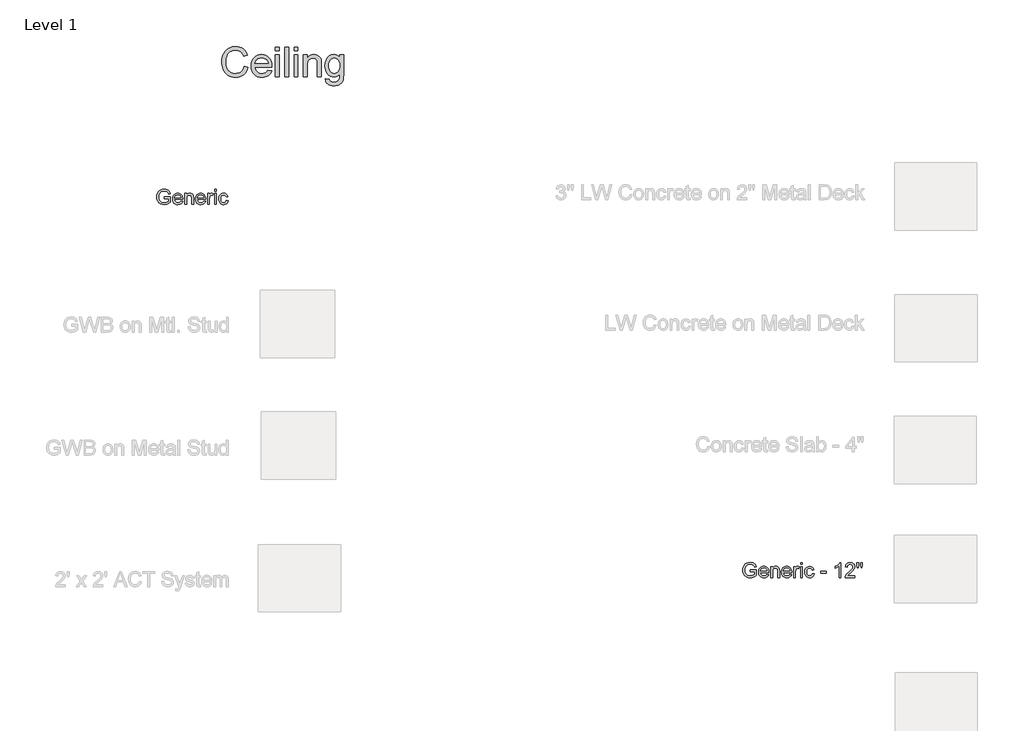
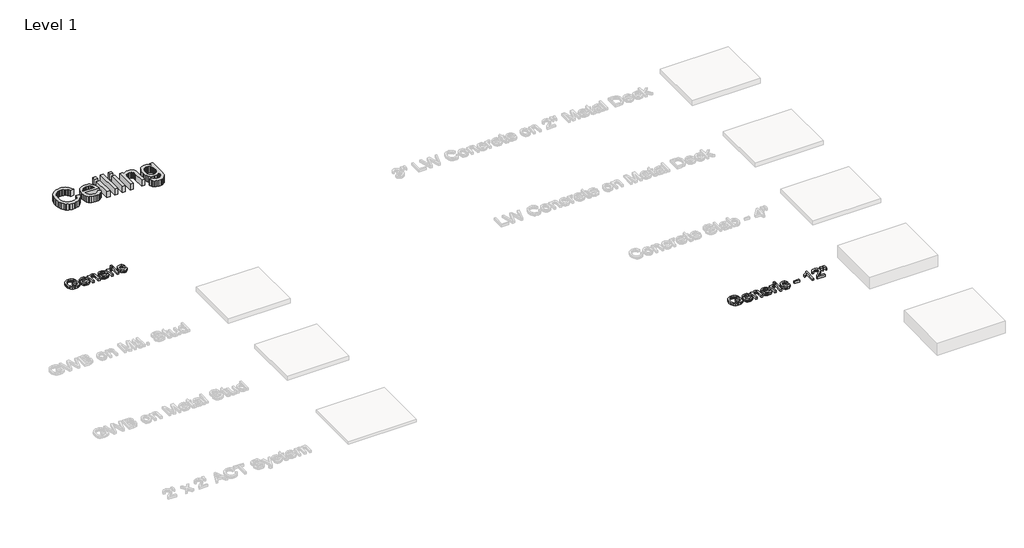
# One storey, part 12 of 42: 3 proxies.
"""IFC4 building model written with IfcOpenShell, lengths in millimetres."""

import ifcopenshell
import ifcopenshell.guid

model = None  # the IFC model being written
_history = None  # IfcOwnerHistory: only IFC2X3 demands one
_inside = {}  # id of a spatial element -> (the spatial element, [elements in it])
_under = {}  # id of a project, library or spatial element -> (it, [spatial elements below it])
_declared = {}  # id of a project -> (the project, [libraries it declares])
_typed = {}  # id of a type object -> (the type object, [elements of that type])
_made_of = {}  # id of a material, layer set ... -> (it, [elements and type objects made of it])


def new_model(schema):
    """Start an empty IFC model of exactly this schema.

    Asked for "IFC4X3", IfcOpenShell would pick the latest addendum, in which some entities
    have other attributes; the version numbers below select the first issue.
    IFC2X3 requires an IfcOwnerHistory on every rooted entity: one is made here for all.
    """
    global model, _history
    if schema == "IFC4X3":
        model = ifcopenshell.file(schema_version=(4, 3, 0, 0))
    else:
        model = ifcopenshell.file(schema=schema)
    _inside.clear()
    _under.clear()
    _declared.clear()
    _typed.clear()
    _made_of.clear()
    _history = None
    if model.schema == "IFC2X3":
        org = make("IfcOrganization", Name="unknown")
        user = make(
            "IfcPersonAndOrganization",
            ThePerson=make("IfcPerson", FamilyName="unknown"),
            TheOrganization=org,
        )
        app = make(
            "IfcApplication",
            ApplicationDeveloper=org,
            Version="unknown",
            ApplicationFullName="unknown",
            ApplicationIdentifier="unknown",
        )
        _history = make(
            "IfcOwnerHistory",
            OwningUser=user,
            OwningApplication=app,
            ChangeAction="ADDED",
            CreationDate=0,
        )
    return model


def make(cls, **values):
    """One entity of the class cls with the attributes given. An attribute that is None is left unset."""
    return model.create_entity(
        cls, **{name: value for name, value in values.items() if value is not None}
    )


def rooted(cls, **values):
    """An entity with a GlobalId (a new one), such as an element, a storey or a relation."""
    return make(cls, GlobalId=ifcopenshell.guid.new(), OwnerHistory=_history, **values)


def si_unit(unit_type, name, prefix=None):
    """IfcSIUnit, for example si_unit("LENGTHUNIT", "METRE", prefix="MILLI")."""
    return make("IfcSIUnit", UnitType=unit_type, Prefix=prefix, Name=name)


def assignment(units):
    """IfcUnitAssignment: the units of a project."""
    return None if units is None else make("IfcUnitAssignment", Units=units)


def point(xyz):
    """IfcCartesianPoint."""
    return None if xyz is None else make("IfcCartesianPoint", Coordinates=xyz)


def direction(xyz):
    """IfcDirection."""
    return None if xyz is None else make("IfcDirection", DirectionRatios=xyz)


def frame(location, z_axis=None, x_axis=None):
    """IfcAxis2Placement3D, a coordinate frame: its origin and axes. An axis left out is left unset."""
    return make(
        "IfcAxis2Placement3D",
        Location=point(location),
        Axis=direction(z_axis),
        RefDirection=direction(x_axis),
    )


def origin():
    """The frame at (0, 0, 0) with its axes left unset."""
    return frame((0.0, 0.0, 0.0))


def origin_with_axes():
    """The frame at (0, 0, 0) with the z axis (0, 0, 1) and the x axis (1, 0, 0) written out."""
    return frame((0.0, 0.0, 0.0), z_axis=(0.0, 0.0, 1.0), x_axis=(1.0, 0.0, 0.0))


def place(relative_to, where):
    """IfcLocalPlacement: puts the frame where relative to a parent placement (None: the world)."""
    return make(
        "IfcLocalPlacement", PlacementRelTo=relative_to, RelativePlacement=where
    )


def context(
    kind, dimensions, precision=None, world=None, true_north=None, identifier=None
):
    """IfcGeometricRepresentationContext, for example the 3D "Model" context."""
    return make(
        "IfcGeometricRepresentationContext",
        ContextIdentifier=identifier,
        ContextType=kind,
        CoordinateSpaceDimension=dimensions,
        Precision=precision,
        WorldCoordinateSystem=world,
        TrueNorth=true_north,
    )


def project(units=None, contexts=None):
    """IfcProject with its units and contexts."""
    return rooted(
        "IfcProject",
        Name="project",
        RepresentationContexts=contexts,
        UnitsInContext=assignment(units),
    )


def spatial(cls, under=None, at=None, **own):
    """A site, building, storey or space (cls), placed at a placement, below another one or the project."""
    s = rooted(cls, ObjectPlacement=at, **own)
    if under is not None:
        _under.setdefault(under.id(), (under, []))[1].append(s)
    return s


def polyline(points):
    """IfcPolyline through the points."""
    return make("IfcPolyline", Points=[point(p) for p in points])


def outline(outer, holes=None, kind="AREA"):
    """IfcArbitraryClosedProfileDef: a profile drawn as a closed curve; with holes, ...WithVoids."""
    if holes is None:
        return make("IfcArbitraryClosedProfileDef", ProfileType=kind, OuterCurve=outer)
    return make(
        "IfcArbitraryProfileDefWithVoids",
        ProfileType=kind,
        OuterCurve=outer,
        InnerCurves=holes,
    )


def extrude(swept, where, along, depth):
    """IfcExtrudedAreaSolid: the profile swept, set in the frame where, extruded along a direction by depth."""
    return make(
        "IfcExtrudedAreaSolid",
        SweptArea=swept,
        Position=where,
        ExtrudedDirection=direction(along),
        Depth=depth,
    )


def shape(context_of_items, identifier, shape_type, items):
    """IfcShapeRepresentation: the items that make up one representation, for example the "Body"."""
    return make(
        "IfcShapeRepresentation",
        ContextOfItems=context_of_items,
        RepresentationIdentifier=identifier,
        RepresentationType=shape_type,
        Items=items,
    )


def made_of(thing, what):
    """Note that an element or type object is made of a material, layer set ...; save() writes the relation."""
    if what is not None:
        _made_of.setdefault(what.id(), (what, []))[1].append(thing)
    return thing


def element(
    cls,
    number,
    at=None,
    inside=None,
    cuts=None,
    type_object=None,
    material=None,
    context=None,
    identifier="Body",
    shape_type=None,
    held_by="IfcProductDefinitionShape",
    body=None,
    shapes=None,
    **own,
):
    """One element of the class cls, such as IfcWall. Its Tag is "e" and its number.

    at: its placement. inside: the storey or other place that contains it. cuts: it is an
    opening in that element (IfcRelVoidsElement). A single representation is given by context,
    identifier, shape_type and body (its items); several are given by shapes. held_by: the class
    of the entity that holds the representations. save() writes the other relations.
    """
    e = rooted(cls, Tag="e%d" % number, ObjectPlacement=at, **own)
    if body is not None:
        shapes = [shape(context, identifier, shape_type, body)]
    if shapes is not None:
        e.Representation = make(held_by, Representations=shapes)
    if inside is not None:
        _inside.setdefault(inside.id(), (inside, []))[1].append(e)
    if cuts is not None:
        rooted(
            "IfcRelVoidsElement", RelatingBuildingElement=cuts, RelatedOpeningElement=e
        )
    if type_object is not None:
        _typed.setdefault(type_object.id(), (type_object, []))[1].append(e)
    return made_of(e, material)


def aggregate(whole, parts):
    """IfcRelAggregates: a whole, such as a stair, and the parts it consists of."""
    return rooted("IfcRelAggregates", RelatingObject=whole, RelatedObjects=parts)


def save(model, path):
    """Write the relations noted so far, then the file.

    IfcRelAggregates (storeys below a building ...), IfcRelContainedInSpatialStructure (elements
    in a storey), IfcRelDefinesByType, IfcRelAssociatesMaterial and IfcRelDeclares: one each for
    every whole, place, type object, material and project.
    """
    for whole, parts in _under.values():
        aggregate(whole, parts)
    for where, things in _inside.values():
        rooted(
            "IfcRelContainedInSpatialStructure",
            RelatedElements=things,
            RelatingStructure=where,
        )
    for kind, things in _typed.values():
        rooted("IfcRelDefinesByType", RelatedObjects=things, RelatingType=kind)
    for what, things in _made_of.values():
        rooted("IfcRelAssociatesMaterial", RelatedObjects=things, RelatingMaterial=what)
    for by, libraries in _declared.values():
        rooted("IfcRelDeclares", RelatingContext=by, RelatedDefinitions=libraries)
    model.write(path)


model = new_model("IFC4")

# Units and contexts
model_context = context("Model", 3, world=origin())
ifc_project = project(units=[si_unit("LENGTHUNIT", "METRE", prefix="MILLI")], contexts=[model_context])

# Site, building, storey
site = spatial("IfcSite", under=ifc_project)
building = spatial("IfcBuilding", under=site)
storey = spatial("IfcBuildingStorey", under=building, Name="Level 1", Elevation=0.0)

# Proxies
placement = place(None, origin())
element("IfcBuildingElementProxy", 1, Name="24\" Arial", ObjectType="24\" Arial", at=placement, inside=storey, context=model_context, shape_type="SweptSolid", body=[
    extrude(outline(polyline([(10519.6706073, -3278.5487239), (10595.8123808, -3298.1790249), (10580.745753, -3345.5306198), (10560.6786034, -3386.9057546), (10535.6109322, -3422.3044295), (10505.5427391, -3451.7266444), (10471.1525338, -3474.8563811), (10433.1188256, -3491.3776216), (10391.4416147, -3501.2903659), (10346.1209008, -3504.5946141), (10299.6894763, -3502.0943532), (10257.8031357, -3494.5935706), (10220.461879, -3482.0922662), (10187.6657061, -3464.5904401), (10158.9638267, -3442.3483424), (10133.90545, -3415.6262234), (10112.4905762, -3384.4240831), (10094.7192053, -3348.7419214), (10080.7632882, -3310.1226503), (10070.7947759, -3270.1091816), (10064.8136686, -3228.7015155), (10062.8199662, -3185.8996518), (10065.0739188, -3139.9747858), (10071.8357767, -3097.0799756), (10083.10554, -3057.2152214), (10098.8832085, -3020.3805231), (10118.8155856, -2987.1846803), (10142.5494746, -2958.2364926), (10170.0848755, -2933.53596), (10201.4217883, -2913.0830825), (10235.4959755, -2897.0451638), (10271.2431997, -2885.5895075), (10308.663461, -2878.7161138), (10347.7567592, -2876.4249825), (10391.3068422, -2879.3899759), (10431.2413063, -2888.284956), (10467.5601515, -2903.1099229), (10500.2633779, -2923.8648766), (10528.8118956, -2950.0014326), (10552.6666151, -2980.9712067), (10571.8275362, -3016.7741989), (10586.2946591, -3057.410409), (10510.1528856, -3075.553566), (10498.162787, -3045.6108508), (10483.7560793, -3020.0273264), (10466.9327627, -2998.8029929), (10447.692837, -2981.9378503), (10425.9247665, -2969.0879966), (10401.5170153, -2959.9095296), (10374.4695836, -2954.4024494), (10344.7824712, -2952.5667561), (10310.6246321, -2954.6022844), (10279.3853132, -2960.7088695), (10251.0645144, -2970.8865114), (10225.6622357, -2985.13521), (10203.4991426, -3002.8136344), (10184.8959004, -3023.2804539), (10169.8525092, -3046.5356684), (10158.3689691, -3072.579278), (10143.813547, -3128.3099999), (10138.9617397, -3185.7509374), (10144.7058334, -3256.0928493), (10151.8859506, -3287.6946596), (10161.9381147, -3316.9170395), (10175.024982, -3343.1790733), (10191.309209, -3365.8998454), (10210.7907956, -3385.0793559), (10233.4697418, -3400.7176047), (10258.2446316, -3412.8517704), (10284.0140489, -3421.5190316), (10310.7779939, -3426.7193883), (10338.5364664, -3428.4528405), (10371.6393626, -3426.0919994), (10402.0932837, -3419.009476), (10429.8982294, -3407.2052704), (10455.0541999, -3390.6793826), (10476.9663374, -3369.5061697), (10495.0397845, -3343.7599889), (10509.2745411, -3313.4408404), (10519.6706073, -3278.5487239)])), origin_with_axes(), (0.0, 0.0, 1.0), 152.4),
    extrude(outline(polyline([(11004.182127, -3361.8287887), (11078.8367565, -3371.3465104), (11067.3903949, -3401.2473997), (11051.9380392, -3427.5977327), (11032.4796892, -3450.3975094), (11009.0153451, -3469.6467297), (10981.7866676, -3484.9364291), (10951.0353178, -3495.857643), (10916.7612956, -3502.4103713), (10878.964601, -3504.5946141), (10831.7198946, -3500.8256334), (10789.6244244, -3489.5186916), (10752.6781903, -3470.6737886), (10720.8811924, -3444.2909243), (10695.31161, -3411.1043761), (10677.0476225, -3371.8484215), (10666.0892301, -3326.5230603), (10662.4364326, -3275.1282927), (10666.1264087, -3221.9907781), (10677.1963369, -3175.1550363), (10695.6462174, -3134.6210673), (10721.47605, -3100.388871), (10753.1893961, -3073.1927249), (10789.289817, -3053.7669062), (10829.7773128, -3042.111415), (10874.6518834, -3038.2262513), (10918.0811359, -3042.1021203), (10957.3556799, -3053.7297276), (10992.4755152, -3073.109073), (11023.440642, -3100.2401566), (11048.7174429, -3134.3979957), (11066.7723007, -3174.8576075), (11077.6052154, -3221.6189921), (11081.2161869, -3274.6821495), (11080.7700437, -3295.2047369), (10738.5782061, -3295.2047369), (10742.9885176, -3325.588948), (10751.7580199, -3352.1995312), (10764.8867132, -3375.0364865), (10782.3745973, -3394.0998138), (10803.2550288, -3409.129263), (10826.5613639, -3419.8645839), (10852.2936026, -3426.3057764), (10880.4517451, -3428.4528405), (10920.9764194, -3424.4747303), (10955.1063746, -3412.5403996), (10982.8416104, -3391.9062764), (11004.182127, -3361.8287887)]), holes=[polyline([(10738.5782061, -3219.0629634), (11005.0744134, -3219.0629634), (10994.7759411, -3178.8357178), (10985.9181396, -3163.0162233), (10974.5879611, -3150.0594811), (10953.8237128, -3134.444469), (10930.1967123, -3123.2908889), (10903.7069596, -3116.5987408), (10874.3544546, -3114.3680248), (10847.581215, -3116.1479503), (10823.0293968, -3121.4877267), (10800.699, -3130.3873542), (10780.5900245, -3142.8468326), (10763.7155873, -3158.2898938), (10751.0888051, -3176.1402693), (10742.7096781, -3196.3979591), (10738.5782061, -3219.0629634)])]), origin_with_axes(), (0.0, 0.0, 1.0), 152.4),
    extrude(outline(polyline([(11157.3579605, -2962.0844777), (11157.3579605, -2885.9427042), (11233.499734, -2885.9427042), (11233.499734, -2962.0844777), (11157.3579605, -2962.0844777)])), origin_with_axes(), (0.0, 0.0, 1.0), 152.4),
    extrude(outline(polyline([(11157.3579605, -3495.0768924), (11157.3579605, -3047.7439729), (11233.499734, -3047.7439729), (11233.499734, -3495.0768924), (11157.3579605, -3495.0768924)])), origin_with_axes(), (0.0, 0.0, 1.0), 152.4),
    extrude(outline(polyline([(11347.7123943, -3495.0768924), (11347.7123943, -2885.9427042), (11423.8541678, -2885.9427042), (11423.8541678, -3495.0768924), (11347.7123943, -3495.0768924)])), origin_with_axes(), (0.0, 0.0, 1.0), 152.4),
    extrude(outline(polyline([(11538.0668281, -2962.0844777), (11538.0668281, -2885.9427042), (11614.2086016, -2885.9427042), (11614.2086016, -2962.0844777), (11538.0668281, -2962.0844777)])), origin_with_axes(), (0.0, 0.0, 1.0), 152.4),
    extrude(outline(polyline([(11538.0668281, -3495.0768924), (11538.0668281, -3047.7439729), (11614.2086016, -3047.7439729), (11614.2086016, -3495.0768924), (11538.0668281, -3495.0768924)])), origin_with_axes(), (0.0, 0.0, 1.0), 152.4),
    extrude(outline(polyline([(11728.4212618, -3495.0768924), (11728.4212618, -3047.7439729), (11804.5630354, -3047.7439729), (11804.5630354, -3110.2040215), (11831.0156095, -3078.713747), (11862.7847235, -3056.2206938), (11899.8703774, -3042.7248619), (11942.2725711, -3038.2262513), (11979.8043681, -3041.8511648), (12014.1759841, -3052.7259054), (12042.840685, -3069.4934542), (12063.2517366, -3090.7967922), (12077.1007652, -3116.5801515), (12086.0793972, -3146.7877643), (12090.0946861, -3220.401393), (12090.0946861, -3495.0768924), (12013.9529125, -3495.0768924), (12013.9529125, -3230.6626867), (12011.7593751, -3191.2905489), (12005.1787629, -3163.2950628), (11993.0399498, -3143.2372079), (11974.1718102, -3127.6779637), (11949.9871306, -3117.6955095), (11921.8986981, -3114.3680248), (11898.778256, -3116.2362494), (11877.3029669, -3121.8409234), (11857.472831, -3131.1820468), (11839.2878481, -3144.2596195), (11824.0957425, -3162.5607855), (11813.2442385, -3187.5726889), (11806.7333362, -3219.2953296), (11804.5630354, -3257.7287077), (11804.5630354, -3495.0768924), (11728.4212618, -3495.0768924)])), origin_with_axes(), (0.0, 0.0, 1.0), 152.4),
    extrude(outline(polyline([(12175.7541813, -3533.1477791), (12251.8959548, -3542.6655008), (12260.2983185, -3566.459805), (12276.5825454, -3582.8183892), (12308.5933203, -3595.5334705), (12350.4936029, -3599.7718309), (12395.1822805, -3594.9757915), (12413.232491, -3588.9807422), (12428.4199492, -3580.5876732), (12451.4706815, -3557.5369409), (12465.5985496, -3526.7530599), (12469.7253742, -3493.998713), (12470.8035536, -3437.9705622), (12445.4663375, -3462.9545817), (12417.1920119, -3480.8003098), (12385.9805769, -3491.5077467), (12351.8320325, -3495.0768924), (12310.0851116, -3490.9221838), (12273.3294179, -3478.458058), (12241.5649512, -3457.6845151), (12214.7917116, -3428.6015549), (12193.5487888, -3393.7094385), (12178.3752726, -3355.5084266), (12169.2711628, -3313.9985194), (12166.2364596, -3269.1797166), (12171.6831245, -3207.704901), (12188.0231194, -3151.1748391), (12200.1340484, -3125.6842613), (12214.6801758, -3103.2702126), (12231.6615015, -3083.9326931), (12251.0780256, -3067.6717027), (12272.6183771, -3054.7893177), (12295.9711855, -3045.5876141), (12321.1364506, -3040.066592), (12348.1141725, -3038.2262513), (12383.721977, -3042.3902545), (12416.0394753, -3054.8822642), (12445.0666675, -3075.7022804), (12470.8035536, -3104.8503031), (12470.8035536, -3047.7439729), (12546.9453272, -3047.7439729), (12546.9453272, -3433.9552734), (12541.7403231, -3523.1281463), (12535.234068, -3556.2961052), (12526.125311, -3581.8517456), (12514.1956276, -3602.4626321), (12499.2265936, -3620.7963294), (12481.2182091, -3636.8528375), (12460.1704739, -3650.6321562), (12436.2971652, -3661.6927898), (12409.8120598, -3669.5932424), (12380.7151577, -3674.3335139), (12349.0064589, -3675.9136045), (12311.7023808, -3673.6875358), (12278.1626359, -3667.0093297), (12248.3872244, -3655.8789862), (12222.3761461, -3640.2965053), (12201.3655896, -3620.2432978), (12186.5917433, -3595.7007742), (12178.0546072, -3566.6689347), (12175.7541813, -3533.1477791)]), holes=[polyline([(12242.3782331, -3263.9747126), (12244.4091141, -3301.6226928), (12250.5017573, -3333.8147133), (12260.6561625, -3360.5507743), (12274.8723298, -3381.8308757), (12292.1557316, -3398.0639821), (12311.5118404, -3409.6590581), (12332.9406562, -3416.6161036), (12356.442179, -3418.9351188), (12379.7113355, -3416.6300456), (12401.0379101, -3409.714826), (12420.4219028, -3398.1894598), (12437.8633137, -3382.0539473), (12452.2746687, -3360.9829755), (12462.5684937, -3334.6512319), (12468.7447886, -3303.0587162), (12470.8035536, -3266.2054286), (12468.6843734, -3230.8904056), (12462.3268328, -3200.1948237), (12451.7309317, -3174.1186829), (12436.8966701, -3152.6619831), (12419.0788259, -3135.9083764), (12399.5321768, -3123.9415144), (12378.2567227, -3116.7613972), (12355.2524637, -3114.3680248), (12332.6339328, -3116.7242186), (12311.7720906, -3123.7928), (12292.6669374, -3135.573769), (12275.318473, -3152.0671255), (12260.907118, -3173.1985125), (12250.6132931, -3198.8935727), (12244.4369981, -3229.152306), (12242.3782331, -3263.9747126)])]), origin_with_axes(), (0.0, 0.0, 1.0), 152.4),
])
element("IfcBuildingElementProxy", 2, Name="8\" Arial", ObjectType="8\" Arial", at=placement, inside=storey, context=model_context, shape_type="SweptSolid", body=[
    extrude(outline(polyline([(8891.7639138, -5976.3008915), (8891.7639138, -5938.2300048), (9015.4942958, -5938.2300048), (9015.4942958, -6052.070879), (8985.4261028, -6072.9838417), (8954.4098554, -6087.985407), (8922.519911, -6097.0198069), (8889.8306266, -6100.0312735), (8847.1217095, -6095.2445287), (8808.5210276, -6080.8842943), (8776.4544848, -6057.4524814), (8753.3479847, -6025.4510012), (8739.3781256, -5987.0640963), (8734.721506, -5944.4760096), (8739.3595363, -5901.5811995), (8753.2736275, -5861.6792666), (8775.8875112, -5828.2092317), (8790.2407746, -5815.1758086), (8806.624919, -5804.6101151), (8844.0637696, -5790.6123721), (8886.7819814, -5785.9464577), (8918.1421308, -5788.6512009), (8946.3420991, -5796.7654304), (8970.0899301, -5809.7035834), (8988.0936673, -5826.8800967), (9001.4129009, -5849.1221944), (9011.107221, -5877.2571002), (8976.0106222, -5887.1466079), (8968.1752322, -5867.0794584), (8958.6482159, -5851.9384734), (8946.0446703, -5840.5246431), (8928.9796928, -5831.6389576), (8908.6337037, -5825.9227478), (8886.1871238, -5824.0173445), (8859.911148, -5826.0714622), (8837.4459787, -5832.2338152), (8818.8752678, -5841.7329476), (8804.2826672, -5853.7974034), (8784.6895448, -5883.1313191), (8775.7666807, -5911.8703771), (8772.7923927, -5942.9145084), (8776.370833, -5979.3216528), (8787.1061538, -6009.27831), (8804.6730425, -6032.5707032), (8828.7461862, -6048.9850552), (8856.9182707, -6058.7165539), (8886.7819814, -6061.9603867), (8913.1509037, -6059.5158938), (8938.8692005, -6052.1824148), (8961.2042446, -6042.0791302), (8977.423409, -6031.32522), (8977.423409, -5976.3008915), (8891.7639138, -5976.3008915)])), origin_with_axes(), (0.0, 0.0, 1.0), 50.8),
    extrude(outline(polyline([(9229.1968906, -6028.6483608), (9266.5242054, -6033.4072217), (9253.0748467, -6061.5328328), (9231.6134996, -6082.5573313), (9202.623486, -6095.662788), (9166.5881276, -6100.0312735), (9142.9657744, -6098.1467832), (9121.9180393, -6092.4933123), (9103.4449223, -6083.0708607), (9087.5464233, -6069.8794286), (9074.7616321, -6053.2861545), (9065.6296384, -6033.6581772), (9060.1504421, -6010.9954966), (9058.3240434, -5985.2981128), (9060.1690314, -5958.7293555), (9065.7039956, -5935.3114846), (9074.9289358, -5915.0445001), (9087.8438521, -5897.928402), (9103.7005251, -5884.3303289), (9121.7507356, -5874.6174196), (9141.9944835, -5868.789674), (9164.4317688, -5866.8470921), (9186.1463951, -5868.7850266), (9205.783667, -5874.5988303), (9223.3435847, -5884.288503), (9238.8261481, -5897.8540448), (9251.4645486, -5914.9329643), (9260.4919775, -5935.1627702), (9265.9084348, -5958.5434625), (9267.7139206, -5985.0750412), (9267.490849, -5995.3363349), (9096.3949302, -5995.3363349), (9102.9848371, -6023.8337321), (9118.2931258, -6044.7838734), (9140.386509, -6057.6662584), (9167.3316996, -6061.9603867), (9187.5940368, -6059.9713316), (9204.6590144, -6054.0041663), (9218.5266323, -6043.6871047), (9229.1968906, -6028.6483608)]), holes=[polyline([(9096.3949302, -5957.2654481), (9229.6430338, -5957.2654481), (9224.4937977, -5937.1518254), (9214.3998077, -5922.763707), (9192.2041833, -5909.3794109), (9164.2830544, -5904.9179789), (9138.6205255, -5908.4778298), (9117.4008394, -5919.1573828), (9102.6502297, -5935.8041011), (9096.3949302, -5957.2654481)])]), origin_with_axes(), (0.0, 0.0, 1.0), 50.8),
    extrude(outline(polyline([(9305.7848073, -6095.2724126), (9305.7848073, -5871.6059529), (9343.8556941, -5871.6059529), (9343.8556941, -5902.8359772), (9357.0819812, -5887.09084), (9372.9665382, -5875.8443134), (9391.5093651, -5869.0963974), (9412.7104619, -5866.8470921), (9431.4763605, -5868.6595489), (9448.6621685, -5874.0969192), (9462.9945189, -5882.4806935), (9473.2000447, -5893.1323625), (9484.613875, -5921.1278486), (9486.6215194, -5957.934663), (9486.6215194, -6095.2724126), (9448.5506327, -6095.2724126), (9448.5506327, -5963.0653098), (9444.1635578, -5929.3814979), (9438.0941513, -5919.3525704), (9428.6600815, -5911.5729483), (9416.5677417, -5906.5817212), (9402.5235254, -5904.9179789), (9380.2256599, -5908.6544282), (9361.2181005, -5919.8637762), (9353.6220477, -5929.0143592), (9348.1962957, -5941.5203109), (9343.8556941, -5976.5983203), (9343.8556941, -6095.2724126), (9305.7848073, -6095.2724126)])), origin_with_axes(), (0.0, 0.0, 1.0), 50.8),
    extrude(outline(polyline([(9695.5652534, -6028.6483608), (9732.8925682, -6033.4072217), (9719.4432095, -6061.5328328), (9697.9818624, -6082.5573313), (9668.9918488, -6095.662788), (9632.9564904, -6100.0312735), (9609.3341372, -6098.1467832), (9588.2864021, -6092.4933123), (9569.813285, -6083.0708607), (9553.9147861, -6069.8794286), (9541.1299949, -6053.2861545), (9531.9980012, -6033.6581772), (9526.5188049, -6010.9954966), (9524.6924062, -5985.2981128), (9526.5373942, -5958.7293555), (9532.0723584, -5935.3114846), (9541.2972986, -5915.0445001), (9554.2122149, -5897.928402), (9570.0688879, -5884.3303289), (9588.1190984, -5874.6174196), (9608.3628463, -5868.789674), (9630.8001316, -5866.8470921), (9652.5147579, -5868.7850266), (9672.1520298, -5874.5988303), (9689.7119475, -5884.288503), (9705.1945109, -5897.8540448), (9717.8329113, -5914.9329643), (9726.8603402, -5935.1627702), (9732.2767976, -5958.5434625), (9734.0822834, -5985.0750412), (9733.8592118, -5995.3363349), (9562.763293, -5995.3363349), (9569.3531999, -6023.8337321), (9584.6614886, -6044.7838734), (9606.7548718, -6057.6662584), (9633.7000624, -6061.9603867), (9653.9623996, -6059.9713316), (9671.0273772, -6054.0041663), (9684.8949951, -6043.6871047), (9695.5652534, -6028.6483608)]), holes=[polyline([(9562.763293, -5957.2654481), (9696.0113966, -5957.2654481), (9690.8621605, -5937.1518254), (9680.7681705, -5922.763707), (9658.5725461, -5909.3794109), (9630.6514172, -5904.9179789), (9604.9888883, -5908.4778298), (9583.7692021, -5919.1573828), (9569.0185925, -5935.8041011), (9562.763293, -5957.2654481)])]), origin_with_axes(), (0.0, 0.0, 1.0), 50.8),
    extrude(outline(polyline([(9772.1531701, -6095.2724126), (9772.1531701, -5871.6059529), (9805.465196, -5871.6059529), (9805.465196, -5904.6949073), (9817.7713128, -5885.5107495), (9829.1107859, -5874.208455), (9840.4874376, -5868.6874328), (9852.9050901, -5866.8470921), (9871.8661763, -5869.7842015), (9891.1246912, -5878.5955298), (9878.4096099, -5912.7254849), (9865.0253138, -5906.8698554), (9851.6410177, -5904.9179789), (9840.2736606, -5906.7954982), (9830.1146081, -5912.4280561), (9821.907432, -5921.3880988), (9816.3957045, -5933.2480723), (9811.7669688, -5954.5142317), (9810.2240569, -5977.7136783), (9810.2240569, -6095.2724126), (9772.1531701, -6095.2724126)])), origin_with_axes(), (0.0, 0.0, 1.0), 50.8),
    extrude(outline(polyline([(9914.9189955, -6095.2724126), (9914.9189955, -5871.6059529), (9952.9898822, -5871.6059529), (9952.9898822, -6095.2724126), (9914.9189955, -6095.2724126)])), origin_with_axes(), (0.0, 0.0, 1.0), 50.8),
    extrude(outline(polyline([(9914.9189955, -5828.7762053), (9914.9189955, -5790.7053186), (9952.9898822, -5790.7053186), (9952.9898822, -5828.7762053), (9914.9189955, -5828.7762053)])), origin_with_axes(), (0.0, 0.0, 1.0), 50.8),
    extrude(outline(polyline([(10152.8620377, -6014.3717783), (10190.9329245, -6019.1306391), (10180.3184341, -6052.9910494), (10160.372115, -6078.5792211), (10132.9714865, -6094.6682604), (10099.994068, -6100.0312735), (10078.6419331, -6098.1607252), (10059.4972776, -6092.5490802), (10042.5601015, -6083.1963385), (10027.8304047, -6070.1025002), (10015.9076923, -6053.5138735), (10007.3914692, -6033.6767665), (10002.2817353, -6010.5911794), (10000.5784907, -5984.257112), (10003.4877162, -5950.3781124), (10012.2153926, -5921.0163128), (10026.9009397, -5897.3056604), (10047.6837773, -5880.3801026), (10072.5469663, -5870.2303447), (10099.4735676, -5866.8470921), (10131.6423516, -5871.4944171), (10157.3606484, -5885.4363923), (10175.8105288, -5907.9294455), (10186.1740636, -5938.2300048), (10148.1031769, -5942.9888656), (10141.1972518, -5926.3793259), (10130.4433417, -5914.4728791), (10116.436304, -5907.3067039), (10099.7709964, -5904.9179789), (10075.1680576, -5909.6210718), (10055.6399978, -5923.7303506), (10042.8970325, -5948.0079767), (10038.6493774, -5983.2161112), (10042.804086, -6018.8982729), (10055.2682118, -6043.2595508), (10074.4430749, -6057.2851777), (10098.7299956, -6061.9603867), (10118.4439484, -6059.0418666), (10134.6073449, -6050.2863062), (10146.3650773, -6035.470634), (10152.8620377, -6014.3717783)])), origin_with_axes(), (0.0, 0.0, 1.0), 50.8),
])
element("IfcBuildingElementProxy", 3, Name="8\" Arial", ObjectType="8\" Arial", at=placement, inside=storey, context=model_context, shape_type="SweptSolid", body=[
    extrude(outline(polyline([(20843.5857887, -13586.9353263), (20843.5857887, -13548.8644395), (20967.3161707, -13548.8644395), (20967.3161707, -13662.7053138), (20937.2479777, -13683.6182765), (20906.2317303, -13698.6198417), (20874.3417859, -13707.6542416), (20841.6525015, -13710.6657082), (20798.9435844, -13705.8789634), (20760.3429025, -13691.518729), (20728.2763597, -13668.0869162), (20705.1698596, -13636.0854359), (20691.2000005, -13597.6985311), (20686.5433808, -13555.1104444), (20691.1814112, -13512.2156342), (20705.0955024, -13472.3137014), (20727.7093861, -13438.8436664), (20742.0626495, -13425.8102433), (20758.4467939, -13415.2445498), (20795.8856445, -13401.2468068), (20838.6038563, -13396.5808925), (20869.9640057, -13399.2856356), (20898.163974, -13407.3998652), (20921.911805, -13420.3380181), (20939.9155422, -13437.5145315), (20953.2347758, -13459.7566291), (20962.9290958, -13487.8915349), (20927.8324971, -13497.7810426), (20919.9971071, -13477.7138931), (20910.4700908, -13462.5729081), (20897.8665452, -13451.1590778), (20880.8015677, -13442.2733923), (20860.4555786, -13436.5571825), (20838.0089987, -13434.6517792), (20811.7330229, -13436.7058969), (20789.2678536, -13442.8682499), (20770.6971427, -13452.3673823), (20756.1045421, -13464.4318381), (20736.5114197, -13493.7657538), (20727.5885556, -13522.5048119), (20724.6142676, -13553.5489431), (20728.1927079, -13589.9560875), (20738.9280287, -13619.9127448), (20756.4949174, -13643.2051379), (20780.5680611, -13659.6194899), (20808.7401455, -13669.3509886), (20838.6038563, -13672.5948215), (20864.9727786, -13670.1503285), (20890.6910754, -13662.8168496), (20913.0261195, -13652.7135649), (20929.2452839, -13641.9596548), (20929.2452839, -13586.9353263), (20843.5857887, -13586.9353263)])), origin_with_axes(), (0.0, 0.0, 1.0), 50.8),
    extrude(outline(polyline([(21181.0187655, -13639.2827956), (21218.3460803, -13644.0416564), (21204.8967216, -13672.1672676), (21183.4353745, -13693.1917661), (21154.4453609, -13706.2972227), (21118.4100025, -13710.6657082), (21094.7876493, -13708.7812179), (21073.7399142, -13703.127747), (21055.2667971, -13693.7052955), (21039.3682982, -13680.5138633), (21026.583507, -13663.9205893), (21017.4515133, -13644.292612), (21011.972317, -13621.6299314), (21010.1459183, -13595.9325475), (21011.9909063, -13569.3637903), (21017.5258705, -13545.9459194), (21026.7508107, -13525.6789349), (21039.665727, -13508.5628367), (21055.5224, -13494.9647636), (21073.5726105, -13485.2518543), (21093.8163584, -13479.4241087), (21116.2536437, -13477.4815268), (21137.96827, -13479.4194614), (21157.6055419, -13485.233265), (21175.1654596, -13494.9229377), (21190.648023, -13508.4884795), (21203.2864234, -13525.5673991), (21212.3138523, -13545.797205), (21217.7303097, -13569.1778973), (21219.5357955, -13595.7094759), (21219.3127239, -13605.9707696), (21048.2168051, -13605.9707696), (21054.806712, -13634.4681668), (21070.1150007, -13655.4183081), (21092.2083839, -13668.3006931), (21119.1535745, -13672.5948215), (21139.4159117, -13670.6057664), (21156.4808893, -13664.638601), (21170.3485072, -13654.3215394), (21181.0187655, -13639.2827956)]), holes=[polyline([(21048.2168051, -13567.8998829), (21181.4649087, -13567.8998829), (21176.3156726, -13547.7862601), (21166.2216826, -13533.3981418), (21144.0260582, -13520.0138456), (21116.1049293, -13515.5524136), (21090.4424004, -13519.1122646), (21069.2227142, -13529.7918175), (21054.4721046, -13546.4385358), (21048.2168051, -13567.8998829)])]), origin_with_axes(), (0.0, 0.0, 1.0), 50.8),
    extrude(outline(polyline([(21257.6066822, -13705.9068474), (21257.6066822, -13482.2403877), (21295.677569, -13482.2403877), (21295.677569, -13513.470412), (21308.9038561, -13497.7252747), (21324.7884131, -13486.4787481), (21343.33124, -13479.7308322), (21364.5323368, -13477.4815268), (21383.2982354, -13479.2939836), (21400.4840434, -13484.7313539), (21414.8163938, -13493.1151283), (21425.0219196, -13503.7667973), (21436.4357499, -13531.7622833), (21438.4433943, -13568.5690977), (21438.4433943, -13705.9068474), (21400.3725076, -13705.9068474), (21400.3725076, -13573.6997445), (21395.9854327, -13540.0159326), (21389.9160262, -13529.9870052), (21380.4819564, -13522.2073831), (21368.3896166, -13517.216156), (21354.3454003, -13515.5524136), (21332.0475348, -13519.2888629), (21313.0399753, -13530.4982109), (21305.4439226, -13539.6487939), (21300.0181706, -13552.1547456), (21295.677569, -13587.2327551), (21295.677569, -13705.9068474), (21257.6066822, -13705.9068474)])), origin_with_axes(), (0.0, 0.0, 1.0), 50.8),
    extrude(outline(polyline([(21647.3871283, -13639.2827956), (21684.714443, -13644.0416564), (21671.2650844, -13672.1672676), (21649.8037373, -13693.1917661), (21620.8137237, -13706.2972227), (21584.7783653, -13710.6657082), (21561.1560121, -13708.7812179), (21540.108277, -13703.127747), (21521.6351599, -13693.7052955), (21505.736661, -13680.5138633), (21492.9518698, -13663.9205893), (21483.8198761, -13644.292612), (21478.3406798, -13621.6299314), (21476.5142811, -13595.9325475), (21478.3592691, -13569.3637903), (21483.8942333, -13545.9459194), (21493.1191735, -13525.6789349), (21506.0340898, -13508.5628367), (21521.8907628, -13494.9647636), (21539.9409733, -13485.2518543), (21560.1847212, -13479.4241087), (21582.6220065, -13477.4815268), (21604.3366328, -13479.4194614), (21623.9739047, -13485.233265), (21641.5338224, -13494.9229377), (21657.0163858, -13508.4884795), (21669.6547862, -13525.5673991), (21678.6822151, -13545.797205), (21684.0986725, -13569.1778973), (21685.9041583, -13595.7094759), (21685.6810867, -13605.9707696), (21514.5851678, -13605.9707696), (21521.1750748, -13634.4681668), (21536.4833634, -13655.4183081), (21558.5767467, -13668.3006931), (21585.5219373, -13672.5948215), (21605.7842745, -13670.6057664), (21622.8492521, -13664.638601), (21636.71687, -13654.3215394), (21647.3871283, -13639.2827956)]), holes=[polyline([(21514.5851678, -13567.8998829), (21647.8332715, -13567.8998829), (21642.6840353, -13547.7862601), (21632.5900454, -13533.3981418), (21610.3944209, -13520.0138456), (21582.4732921, -13515.5524136), (21556.8107632, -13519.1122646), (21535.591077, -13529.7918175), (21520.8404674, -13546.4385358), (21514.5851678, -13567.8998829)])]), origin_with_axes(), (0.0, 0.0, 1.0), 50.8),
    extrude(outline(polyline([(21723.975045, -13705.9068474), (21723.975045, -13482.2403877), (21757.2870709, -13482.2403877), (21757.2870709, -13515.329342), (21769.5931876, -13496.1451842), (21780.9326608, -13484.8428897), (21792.3093125, -13479.3218675), (21804.726965, -13477.4815268), (21823.6880512, -13480.4186363), (21842.9465661, -13489.2299645), (21830.2314848, -13523.3599197), (21816.8471887, -13517.5042901), (21803.4628926, -13515.5524136), (21792.0955355, -13517.4299329), (21781.936483, -13523.0624909), (21773.7293069, -13532.0225335), (21768.2175794, -13543.8825071), (21763.5888437, -13565.1486665), (21762.0459318, -13588.3481131), (21762.0459318, -13705.9068474), (21723.975045, -13705.9068474)])), origin_with_axes(), (0.0, 0.0, 1.0), 50.8),
    extrude(outline(polyline([(21866.7408704, -13705.9068474), (21866.7408704, -13482.2403877), (21904.8117571, -13482.2403877), (21904.8117571, -13705.9068474), (21866.7408704, -13705.9068474)])), origin_with_axes(), (0.0, 0.0, 1.0), 50.8),
    extrude(outline(polyline([(21866.7408704, -13439.4106401), (21866.7408704, -13401.3397533), (21904.8117571, -13401.3397533), (21904.8117571, -13439.4106401), (21866.7408704, -13439.4106401)])), origin_with_axes(), (0.0, 0.0, 1.0), 50.8),
    extrude(outline(polyline([(22104.6839126, -13625.006213), (22142.7547994, -13629.7650739), (22132.140309, -13663.6254841), (22112.1939899, -13689.2136558), (22084.7933614, -13705.3026951), (22051.8159429, -13710.6657082), (22030.463808, -13708.7951599), (22011.3191525, -13703.1835149), (21994.3819763, -13693.8307733), (21979.6522796, -13680.7369349), (21967.7295672, -13664.1483082), (21959.2133441, -13644.3112013), (21954.1036102, -13621.2256141), (21952.4003656, -13594.8915467), (21955.309591, -13561.0125472), (21964.0372675, -13531.6507475), (21978.7228146, -13507.9400952), (21999.5056522, -13491.0145374), (22024.3688412, -13480.8647795), (22051.2954425, -13477.4815268), (22083.4642265, -13482.1288519), (22109.1825232, -13496.070827), (22127.6324037, -13518.5638802), (22137.9959385, -13548.8644395), (22099.9250518, -13553.6233003), (22093.0191267, -13537.0137606), (22082.2652166, -13525.1073139), (22068.2581789, -13517.9411387), (22051.5928713, -13515.5524136), (22026.9899325, -13520.2555065), (22007.4618727, -13534.3647854), (21994.7189074, -13558.6424114), (21990.4712523, -13593.8505459), (21994.6259609, -13629.5327076), (22007.0900867, -13653.8939855), (22026.2649498, -13667.9196125), (22050.5518705, -13672.5948215), (22070.2658233, -13669.6763013), (22086.4292198, -13660.920741), (22098.1869522, -13646.1050687), (22104.6839126, -13625.006213)])), origin_with_axes(), (0.0, 0.0, 1.0), 50.8),
    extrude(outline(polyline([(22276.002903, -13615.4884913), (22276.002903, -13577.4176046), (22394.9744241, -13577.4176046), (22394.9744241, -13615.4884913), (22276.002903, -13615.4884913)])), origin_with_axes(), (0.0, 0.0, 1.0), 50.8),
    extrude(outline(polyline([(22690.0237965, -13705.9068474), (22651.9529098, -13705.9068474), (22651.9529098, -13468.5586627), (22615.8896674, -13494.2490756), (22575.8111362, -13513.470412), (22575.8111362, -13477.4815268), (22605.7120256, -13461.2158892), (22631.6162154, -13441.8644277), (22652.0365616, -13421.2860724), (22665.4859203, -13401.3397533), (22690.0237965, -13401.3397533), (22690.0237965, -13705.9068474)])), origin_with_axes(), (0.0, 0.0, 1.0), 50.8),
    extrude(outline(polyline([(22975.5554472, -13667.8359606), (22975.5554472, -13705.9068474), (22775.6832917, -13705.9068474), (22779.7729378, -13679.6587555), (22789.1605343, -13659.1454628), (22802.8980272, -13639.245617), (22822.7699891, -13618.4163061), (22850.5609928, -13595.1146183), (22891.6433462, -13558.6238221), (22916.2927582, -13531.6879261), (22928.6174643, -13509.8269091), (22932.7256996, -13488.5607497), (22928.8498305, -13469.4974224), (22917.2222233, -13453.650044), (22899.3486111, -13442.9704911), (22876.7347275, -13439.4106401), (22852.9868965, -13442.8868392), (22834.5370161, -13453.3154366), (22822.6305693, -13469.8785031), (22818.5130393, -13491.7581094), (22780.4421526, -13486.9992485), (22783.7161931, -13467.3457109), (22789.6717401, -13450.1738449), (22798.3087937, -13435.4836504), (22809.6273538, -13423.2751275), (22823.3671703, -13413.6784013), (22839.267993, -13406.8235969), (22877.5526567, -13401.3397533), (22897.9567373, -13402.8640759), (22916.1161599, -13407.4370438), (22932.0309245, -13415.0586568), (22945.7010311, -13425.7289151), (22956.6803365, -13438.6577734), (22964.5226975, -13453.0551864), (22969.2281142, -13468.9211541), (22970.7965864, -13486.2556765), (22969.10496, -13504.463896), (22964.0300811, -13522.3560975), (22955.0235652, -13540.5550223), (22941.5370279, -13559.6834122), (22920.0385022, -13582.5203675), (22886.9960212, -13611.8449885), (22843.19963, -13648.4659098), (22826.0231166, -13667.8359606), (22975.5554472, -13667.8359606)])), origin_with_axes(), (0.0, 0.0, 1.0), 50.8),
    extrude(outline(polyline([(23022.920984, -13510.7935527), (23013.626334, -13451.977007), (23013.626334, -13401.3397533), (23051.6972207, -13401.3397533), (23051.6972207, -13451.977007), (23043.3692142, -13510.7935527), (23022.920984, -13510.7935527)])), origin_with_axes(), (0.0, 0.0, 1.0), 50.8),
    extrude(outline(polyline([(23098.839686, -13510.7935527), (23089.7681075, -13451.977007), (23089.7681075, -13401.3397533), (23127.8389942, -13401.3397533), (23127.8389942, -13451.977007), (23118.9161302, -13510.7935527), (23098.839686, -13510.7935527)])), origin_with_axes(), (0.0, 0.0, 1.0), 50.8),
])

save(model, "model.ifc")

# Revit data of these elements
# Element 1 (IfcBuildingElementProxy, "24\" Arial")
#   Phase Created = New Construction
# Elements 2, 3 (IfcBuildingElementProxy, "8\" Arial")
#   Phase Created = New Construction
